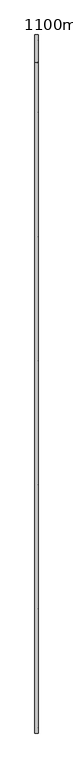
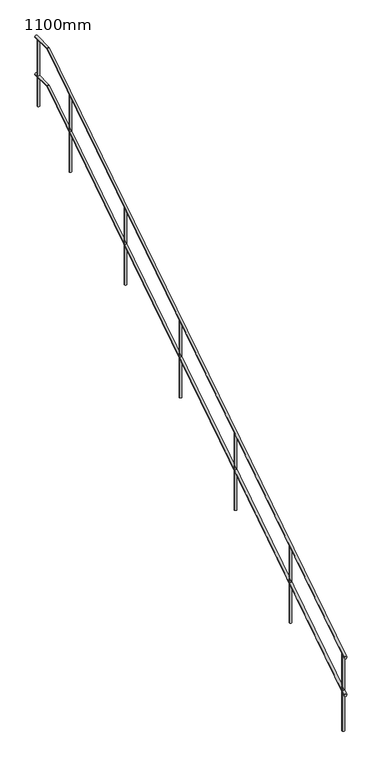
"""IFC4 building model written with IfcOpenShell, lengths in millimetres: railing geometry, 1100mm."""

import ifcopenshell
import ifcopenshell.guid

model = None  # the IFC model being written
_history = None  # IfcOwnerHistory: only IFC2X3 demands one
_inside = {}  # id of a spatial element -> (the spatial element, [elements in it])
_under = {}  # id of a project, library or spatial element -> (it, [spatial elements below it])
_declared = {}  # id of a project -> (the project, [libraries it declares])
_typed = {}  # id of a type object -> (the type object, [elements of that type])
_made_of = {}  # id of a material, layer set ... -> (it, [elements and type objects made of it])


def new_model(schema):
    """Start an empty IFC model of exactly this schema.

    Asked for "IFC4X3", IfcOpenShell would pick the latest addendum, in which some entities
    have other attributes; the version numbers below select the first issue.
    IFC2X3 requires an IfcOwnerHistory on every rooted entity: one is made here for all.
    """
    global model, _history
    if schema == "IFC4X3":
        model = ifcopenshell.file(schema_version=(4, 3, 0, 0))
    else:
        model = ifcopenshell.file(schema=schema)
    _inside.clear()
    _under.clear()
    _declared.clear()
    _typed.clear()
    _made_of.clear()
    _history = None
    if model.schema == "IFC2X3":
        org = make("IfcOrganization", Name="unknown")
        user = make(
            "IfcPersonAndOrganization",
            ThePerson=make("IfcPerson", FamilyName="unknown"),
            TheOrganization=org,
        )
        app = make(
            "IfcApplication",
            ApplicationDeveloper=org,
            Version="unknown",
            ApplicationFullName="unknown",
            ApplicationIdentifier="unknown",
        )
        _history = make(
            "IfcOwnerHistory",
            OwningUser=user,
            OwningApplication=app,
            ChangeAction="ADDED",
            CreationDate=0,
        )
    return model


def make(cls, **values):
    """One entity of the class cls with the attributes given. An attribute that is None is left unset."""
    return model.create_entity(
        cls, **{name: value for name, value in values.items() if value is not None}
    )


def rooted(cls, **values):
    """An entity with a GlobalId (a new one), such as an element, a storey or a relation."""
    return make(cls, GlobalId=ifcopenshell.guid.new(), OwnerHistory=_history, **values)


def si_unit(unit_type, name, prefix=None):
    """IfcSIUnit, for example si_unit("LENGTHUNIT", "METRE", prefix="MILLI")."""
    return make("IfcSIUnit", UnitType=unit_type, Prefix=prefix, Name=name)


def assignment(units):
    """IfcUnitAssignment: the units of a project."""
    return None if units is None else make("IfcUnitAssignment", Units=units)


def point(xyz):
    """IfcCartesianPoint."""
    return None if xyz is None else make("IfcCartesianPoint", Coordinates=xyz)


def direction(xyz):
    """IfcDirection."""
    return None if xyz is None else make("IfcDirection", DirectionRatios=xyz)


def frame(location, z_axis=None, x_axis=None):
    """IfcAxis2Placement3D, a coordinate frame: its origin and axes. An axis left out is left unset."""
    return make(
        "IfcAxis2Placement3D",
        Location=point(location),
        Axis=direction(z_axis),
        RefDirection=direction(x_axis),
    )


def frame_2d(location, x_axis=None):
    """IfcAxis2Placement2D, a coordinate frame in the plane: its origin and x axis."""
    return make(
        "IfcAxis2Placement2D", Location=point(location), RefDirection=direction(x_axis)
    )


def origin():
    """The frame at (0, 0, 0) with its axes left unset."""
    return frame((0.0, 0.0, 0.0))


def place(relative_to, where):
    """IfcLocalPlacement: puts the frame where relative to a parent placement (None: the world)."""
    return make(
        "IfcLocalPlacement", PlacementRelTo=relative_to, RelativePlacement=where
    )


def context(
    kind, dimensions, precision=None, world=None, true_north=None, identifier=None
):
    """IfcGeometricRepresentationContext, for example the 3D "Model" context."""
    return make(
        "IfcGeometricRepresentationContext",
        ContextIdentifier=identifier,
        ContextType=kind,
        CoordinateSpaceDimension=dimensions,
        Precision=precision,
        WorldCoordinateSystem=world,
        TrueNorth=true_north,
    )


def project(units=None, contexts=None):
    """IfcProject with its units and contexts."""
    return rooted(
        "IfcProject",
        Name="project",
        RepresentationContexts=contexts,
        UnitsInContext=assignment(units),
    )


def spatial(cls, under=None, at=None, **own):
    """A site, building, storey or space (cls), placed at a placement, below another one or the project."""
    s = rooted(cls, ObjectPlacement=at, **own)
    if under is not None:
        _under.setdefault(under.id(), (under, []))[1].append(s)
    return s


def circle_curve(where, radius):
    """IfcCircle in the frame where."""
    return make("IfcCircle", Position=where, Radius=radius)


def ellipse_curve(where, semi_axis1, semi_axis2):
    """IfcEllipse in the frame where."""
    return make(
        "IfcEllipse", Position=where, SemiAxis1=semi_axis1, SemiAxis2=semi_axis2
    )


def trimmed(basis, trim1, trim2, sense, master):
    """IfcTrimmedCurve: the piece of a basis curve between two trims."""
    return make(
        "IfcTrimmedCurve",
        BasisCurve=basis,
        Trim1=trim1,
        Trim2=trim2,
        SenseAgreement=sense,
        MasterRepresentation=master,
    )


def segment(curve, same_sense, transition):
    """IfcCompositeCurveSegment."""
    return make(
        "IfcCompositeCurveSegment",
        Transition=transition,
        SameSense=same_sense,
        ParentCurve=curve,
    )


def composite_curve(segments, self_intersect=None):
    """IfcCompositeCurve: segments joined end to end."""
    return make("IfcCompositeCurve", Segments=segments, SelfIntersect=self_intersect)


def outline(outer, holes=None, kind="AREA"):
    """IfcArbitraryClosedProfileDef: a profile drawn as a closed curve; with holes, ...WithVoids."""
    if holes is None:
        return make("IfcArbitraryClosedProfileDef", ProfileType=kind, OuterCurve=outer)
    return make(
        "IfcArbitraryProfileDefWithVoids",
        ProfileType=kind,
        OuterCurve=outer,
        InnerCurves=holes,
    )


def extrude(swept, where, along, depth):
    """IfcExtrudedAreaSolid: the profile swept, set in the frame where, extruded along a direction by depth."""
    return make(
        "IfcExtrudedAreaSolid",
        SweptArea=swept,
        Position=where,
        ExtrudedDirection=direction(along),
        Depth=depth,
    )


def shape(context_of_items, identifier, shape_type, items):
    """IfcShapeRepresentation: the items that make up one representation, for example the "Body"."""
    return make(
        "IfcShapeRepresentation",
        ContextOfItems=context_of_items,
        RepresentationIdentifier=identifier,
        RepresentationType=shape_type,
        Items=items,
    )


def source(mapping_origin, context_of_items, identifier, shape_type, items):
    """IfcRepresentationMap: a shape defined once, which mapped items show again and again."""
    return make(
        "IfcRepresentationMap",
        MappingOrigin=mapping_origin,
        MappedRepresentation=shape(context_of_items, identifier, shape_type, items),
    )


def transform(
    local_origin,
    x_axis=None,
    y_axis=None,
    z_axis=None,
    scale=None,
    scale2=None,
    scale3=None,
    uniform=True,
):
    """IfcCartesianTransformationOperator3D, or its non-uniform kind. x_axis, y_axis, z_axis: its Axis1, 2, 3."""
    if uniform:
        return make(
            "IfcCartesianTransformationOperator3D",
            Axis1=direction(x_axis),
            Axis2=direction(y_axis),
            LocalOrigin=point(local_origin),
            Scale=scale,
            Axis3=direction(z_axis),
        )
    return make(
        "IfcCartesianTransformationOperator3DnonUniform",
        Axis1=direction(x_axis),
        Axis2=direction(y_axis),
        LocalOrigin=point(local_origin),
        Scale=scale,
        Axis3=direction(z_axis),
        Scale2=scale2,
        Scale3=scale3,
    )


def mapped(mapping_source, mapping_target):
    """IfcMappedItem: shows the shape of a source again, moved by a transform."""
    return make(
        "IfcMappedItem", MappingSource=mapping_source, MappingTarget=mapping_target
    )


def made_of(thing, what):
    """Note that an element or type object is made of a material, layer set ...; save() writes the relation."""
    if what is not None:
        _made_of.setdefault(what.id(), (what, []))[1].append(thing)
    return thing


def element(
    cls,
    number,
    at=None,
    inside=None,
    cuts=None,
    type_object=None,
    material=None,
    context=None,
    identifier="Body",
    shape_type=None,
    held_by="IfcProductDefinitionShape",
    body=None,
    shapes=None,
    **own,
):
    """One element of the class cls, such as IfcWall. Its Tag is "e" and its number.

    at: its placement. inside: the storey or other place that contains it. cuts: it is an
    opening in that element (IfcRelVoidsElement). A single representation is given by context,
    identifier, shape_type and body (its items); several are given by shapes. held_by: the class
    of the entity that holds the representations. save() writes the other relations.
    """
    e = rooted(cls, Tag="e%d" % number, ObjectPlacement=at, **own)
    if body is not None:
        shapes = [shape(context, identifier, shape_type, body)]
    if shapes is not None:
        e.Representation = make(held_by, Representations=shapes)
    if inside is not None:
        _inside.setdefault(inside.id(), (inside, []))[1].append(e)
    if cuts is not None:
        rooted(
            "IfcRelVoidsElement", RelatingBuildingElement=cuts, RelatedOpeningElement=e
        )
    if type_object is not None:
        _typed.setdefault(type_object.id(), (type_object, []))[1].append(e)
    return made_of(e, material)


def aggregate(whole, parts):
    """IfcRelAggregates: a whole, such as a stair, and the parts it consists of."""
    return rooted("IfcRelAggregates", RelatingObject=whole, RelatedObjects=parts)


def save(model, path):
    """Write the relations noted so far, then the file.

    IfcRelAggregates (storeys below a building ...), IfcRelContainedInSpatialStructure (elements
    in a storey), IfcRelDefinesByType, IfcRelAssociatesMaterial and IfcRelDeclares: one each for
    every whole, place, type object, material and project.
    """
    for whole, parts in _under.values():
        aggregate(whole, parts)
    for where, things in _inside.values():
        rooted(
            "IfcRelContainedInSpatialStructure",
            RelatedElements=things,
            RelatingStructure=where,
        )
    for kind, things in _typed.values():
        rooted("IfcRelDefinesByType", RelatedObjects=things, RelatingType=kind)
    for what, things in _made_of.values():
        rooted("IfcRelAssociatesMaterial", RelatedObjects=things, RelatingMaterial=what)
    for by, libraries in _declared.values():
        rooted("IfcRelDeclares", RelatingContext=by, RelatedDefinitions=libraries)
    model.write(path)


def plane_surface(at):
    """IfcPlane: the flat surface through the origin of the frame at, square to its z axis."""
    return make("IfcPlane", Position=at)


def cylinder_surface(at, radius):
    """IfcCylindricalSurface: all points at the distance radius from the z axis of the frame at."""
    return make("IfcCylindricalSurface", Position=at, Radius=radius)


def advanced_brep(points, edges, surfaces, faces):
    """IfcAdvancedBrep: a solid bounded by faces that lie on surfaces and meet in shared edges.

    An edge is (start, end): straight between two places in points (the first is 0);
    or (start, end, curve); or (start, end, curve, False) where it runs against its curve.
    A face is (place in surfaces, loops), or (place, loops, False) where it looks against
    its surface's normal. A loop lists edges by number (the first is 1), with a minus sign
    where the edge is run from its end to its start. The first loop is the outer one.
    """
    corners = [point(p) for p in points]
    vertices = [make("IfcVertexPoint", VertexGeometry=c) for c in corners]
    made = []
    for start, end, *more in edges:
        made.append(
            make(
                "IfcEdgeCurve",
                EdgeStart=vertices[start],
                EdgeEnd=vertices[end],
                EdgeGeometry=more[0] if more else make("IfcPolyline", Points=[corners[start], corners[end]]),
                SameSense=more[1] if len(more) > 1 else True,
            )
        )
    hull = []
    for where, loops, *sense in faces:
        bounds = []
        for j, loop in enumerate(loops):
            ring = [make("IfcOrientedEdge", EdgeElement=made[abs(k) - 1], Orientation=k > 0) for k in loop]
            bounds.append(
                make(
                    "IfcFaceOuterBound" if j == 0 else "IfcFaceBound",
                    Bound=make("IfcEdgeLoop", EdgeList=ring),
                    Orientation=True,
                )
            )
        hull.append(make("IfcAdvancedFace", Bounds=bounds, FaceSurface=surfaces[where], SameSense=sense[0] if sense else True))
    return make("IfcAdvancedBrep", Outer=make("IfcClosedShell", CfsFaces=hull))


def railing_1100mm_756f1f54(model_context):
    return source(origin(), model_context, "Body", "SolidModel", [
        advanced_brep(
        [(17846.6097182, 11187.7630152, 456.1549882), (17816.6097182, 11187.7630152, 456.1549882), (17846.6097182, 17937.7630152, 4635.0), (17816.6097182, 17937.7630152, 4635.0), (17846.6097182, 17672.1776886, 4635.0), (17816.6097182, 17672.1776886, 4635.0)],
        [
            (0, 1, ellipse_curve(frame((17831.6097182, 11187.7630152, 456.1549882), z_axis=(0.0, -1.0, 0.0), x_axis=(0.0, 0.0, -1.0)), 17.8450118, 15.0)),
            (1, 0, ellipse_curve(frame((17831.6097182, 11187.7630152, 456.1549882), z_axis=(0.0, -1.0, 0.0), x_axis=(0.0, 0.0, -1.0)), 17.8450118, 15.0)),
            (2, 3, circle_curve(frame((17831.6097182, 17937.7630152, 4635.0), z_axis=(0.0, 1.0, 0.0), x_axis=(-1.0, 0.0, 0.0)), 15.0)),
            (3, 2, circle_curve(frame((17831.6097182, 17937.7630152, 4635.0), z_axis=(0.0, 1.0, 0.0), x_axis=(-1.0, 0.0, 0.0)), 15.0)),
            (0, 4),
            (4, 5, ellipse_curve(frame((17831.6097182, 17672.1776886, 4635.0), z_axis=(0.0, -0.9593151294266218, -0.28233753284532276), x_axis=(0.0, 0.282337532845322, -0.9593151294266221)), 15.6361549, 15.0)),
            (5, 1),
            (5, 4, ellipse_curve(frame((17831.6097182, 17672.1776886, 4635.0), z_axis=(0.0, -0.9593151294266218, -0.28233753284532276), x_axis=(0.0, 0.282337532845322, -0.9593151294266221)), 15.6361549, 15.0)),
            (4, 2),
            (3, 5),
        ],
        [
            plane_surface(frame((17831.6097182, 11187.7630152, 474.0), z_axis=(0.0, -1.0, 0.0), x_axis=(0.0, 0.0, 1.0))),
            plane_surface(frame((17831.6097182, 17937.7630152, 4650.0), z_axis=(0.0, 1.0, 0.0), x_axis=(0.0, 0.0, 1.0))),
            cylinder_surface(frame((17831.6097182, 11195.8885352, 461.3914345), z_axis=(0.0, -0.8405710350936326, -0.5417013337270078), x_axis=(-1.0, 0.0, 0.0)), 15.0),
            cylinder_surface(frame((17831.6097182, 17667.7630152, 4635.0), z_axis=(0.0, -1.0, 0.0), x_axis=(-1.0, 0.0, 0.0)), 15.0),
        ],
        [
            (0, [[1, 2]]),
            (1, [[3, 4]]),
            (2, [[-1, 5, 6, 7]]),
            (2, [[-2, -7, 8, -5]]),
            (3, [[-6, 9, -4, 10]]),
            (3, [[-8, -10, -3, -9]]),
        ],
    ),
        advanced_brep(
        [(17846.6097182, 11187.7630152, 956.1549882), (17816.6097182, 11187.7630152, 956.1549882), (17846.6097182, 17672.1776886, 5135.0), (17816.6097182, 17672.1776886, 5135.0), (17846.6097182, 17937.7630152, 5135.0), (17816.6097182, 17937.7630152, 5135.0)],
        [
            (0, 1, ellipse_curve(frame((17831.6097182, 11187.7630152, 956.1549882), z_axis=(0.0, -1.0, 0.0), x_axis=(0.0, 0.0, -1.0)), 17.8450118, 15.0)),
            (1, 0, ellipse_curve(frame((17831.6097182, 11187.7630152, 956.1549882), z_axis=(0.0, -1.0, 0.0), x_axis=(0.0, 0.0, -1.0)), 17.8450118, 15.0)),
            (0, 2),
            (2, 3, ellipse_curve(frame((17831.6097182, 17672.1776886, 5135.0), z_axis=(0.0, -0.9593151294266218, -0.28233753284532276), x_axis=(0.0, 0.282337532845322, -0.9593151294266221)), 15.6361549, 15.0)),
            (3, 1),
            (3, 2, ellipse_curve(frame((17831.6097182, 17672.1776886, 5135.0), z_axis=(0.0, -0.9593151294266218, -0.28233753284532276), x_axis=(0.0, 0.282337532845322, -0.9593151294266221)), 15.6361549, 15.0)),
            (4, 5, circle_curve(frame((17831.6097182, 17937.7630152, 5135.0), z_axis=(0.0, 1.0, 0.0), x_axis=(-1.0, 0.0, 0.0)), 15.0)),
            (5, 4, circle_curve(frame((17831.6097182, 17937.7630152, 5135.0), z_axis=(0.0, 1.0, 0.0), x_axis=(-1.0, 0.0, 0.0)), 15.0)),
            (2, 4),
            (5, 3),
        ],
        [
            plane_surface(frame((17831.6097182, 11187.7630152, 974.0), z_axis=(0.0, -1.0, 0.0), x_axis=(0.0, 0.0, 1.0))),
            cylinder_surface(frame((17831.6097182, 11195.8885352, 961.3914345), z_axis=(0.0, -0.8405710350936326, -0.5417013337270078), x_axis=(-1.0, 0.0, 0.0)), 15.0),
            plane_surface(frame((17831.6097182, 17937.7630152, 5150.0), z_axis=(0.0, 1.0, 0.0), x_axis=(0.0, 0.0, 1.0))),
            cylinder_surface(frame((17831.6097182, 17667.7630152, 5135.0), z_axis=(0.0, -1.0, 0.0), x_axis=(-1.0, 0.0, 0.0)), 15.0),
        ],
        [
            (0, [[1, 2]]),
            (1, [[-1, 3, 4, 5]]),
            (1, [[-2, -5, 6, -3]]),
            (2, [[7, 8]]),
            (3, [[-4, 9, -8, 10]]),
            (3, [[-6, -10, -7, -9]]),
        ],
    ),
        extrude(outline(composite_curve([segment(trimmed(circle_curve(frame_2d((17831.6097182, 17187.7630152)), 15.0), [point((17816.6097182, 17187.7630152))], [point((17846.6097182, 17187.7630152))], False, "CARTESIAN"), True, "CONTINUOUS"), segment(trimmed(circle_curve(frame_2d((17831.6097182, 17187.7630152)), 15.0), [point((17846.6097182, 17187.7630152))], [point((17816.6097182, 17187.7630152))], False, "CARTESIAN"), True, "CONTINUOUS")], self_intersect=False)), frame((0.0, 0.0, 3790.4451685), z_axis=(0.0, 0.0, 1.0), x_axis=(1.0, 0.0, 0.0)), (0.0, 0.0, 1.0), 1020.2214982),
        extrude(outline(composite_curve([segment(trimmed(circle_curve(frame_2d((17831.6097182, 15987.7630152)), 15.0), [point((17816.6097182, 15987.7630152))], [point((17846.6097182, 15987.7630152))], False, "CARTESIAN"), True, "CONTINUOUS"), segment(trimmed(circle_curve(frame_2d((17831.6097182, 15987.7630152)), 15.0), [point((17846.6097182, 15987.7630152))], [point((17816.6097182, 15987.7630152))], False, "CARTESIAN"), True, "CONTINUOUS")], self_intersect=False)), frame((0.0, 0.0, 3017.1118351), z_axis=(0.0, 0.0, 1.0), x_axis=(1.0, 0.0, 0.0)), (0.0, 0.0, 1.0), 1020.2214982),
        extrude(outline(composite_curve([segment(trimmed(circle_curve(frame_2d((17831.6097182, 14787.7630152)), 15.0), [point((17816.6097182, 14787.7630152))], [point((17846.6097182, 14787.7630152))], False, "CARTESIAN"), True, "CONTINUOUS"), segment(trimmed(circle_curve(frame_2d((17831.6097182, 14787.7630152)), 15.0), [point((17846.6097182, 14787.7630152))], [point((17816.6097182, 14787.7630152))], False, "CARTESIAN"), True, "CONTINUOUS")], self_intersect=False)), frame((0.0, 0.0, 2243.7785018), z_axis=(0.0, 0.0, 1.0), x_axis=(1.0, 0.0, 0.0)), (0.0, 0.0, 1.0), 1020.2214982),
        extrude(outline(composite_curve([segment(trimmed(circle_curve(frame_2d((17831.6097182, 13587.7630152)), 15.0), [point((17816.6097182, 13587.7630152))], [point((17846.6097182, 13587.7630152))], False, "CARTESIAN"), True, "CONTINUOUS"), segment(trimmed(circle_curve(frame_2d((17831.6097182, 13587.7630152)), 15.0), [point((17846.6097182, 13587.7630152))], [point((17816.6097182, 13587.7630152))], False, "CARTESIAN"), True, "CONTINUOUS")], self_intersect=False)), frame((0.0, 0.0, 1470.4451685), z_axis=(0.0, 0.0, 1.0), x_axis=(1.0, 0.0, 0.0)), (0.0, 0.0, 1.0), 1020.2214982),
        extrude(outline(composite_curve([segment(trimmed(circle_curve(frame_2d((17831.6097182, 12387.7630152)), 15.0), [point((17816.6097182, 12387.7630152))], [point((17846.6097182, 12387.7630152))], False, "CARTESIAN"), True, "CONTINUOUS"), segment(trimmed(circle_curve(frame_2d((17831.6097182, 12387.7630152)), 15.0), [point((17846.6097182, 12387.7630152))], [point((17816.6097182, 12387.7630152))], False, "CARTESIAN"), True, "CONTINUOUS")], self_intersect=False)), frame((0.0, 0.0, 697.1118351), z_axis=(0.0, 0.0, 1.0), x_axis=(1.0, 0.0, 0.0)), (0.0, 0.0, 1.0), 1020.2214982),
        extrude(outline(composite_curve([segment(trimmed(circle_curve(frame_2d((17831.6097182, 17887.7630152)), 15.0), [point((17816.6097182, 17887.7630152))], [point((17846.6097182, 17887.7630152))], False, "CARTESIAN"), True, "CONTINUOUS"), segment(trimmed(circle_curve(frame_2d((17831.6097182, 17887.7630152)), 15.0), [point((17846.6097182, 17887.7630152))], [point((17816.6097182, 17887.7630152))], False, "CARTESIAN"), True, "CONTINUOUS")], self_intersect=False)), frame((0.0, 0.0, 4241.5562796), z_axis=(0.0, 0.0, 1.0), x_axis=(1.0, 0.0, 0.0)), (0.0, 0.0, 1.0), 878.4437204),
        extrude(outline(composite_curve([segment(trimmed(circle_curve(frame_2d((17831.6097182, 11237.7630152)), 15.0), [point((17816.6097182, 11237.7630152))], [point((17846.6097182, 11237.7630152))], False, "CARTESIAN"), True, "CONTINUOUS"), segment(trimmed(circle_curve(frame_2d((17831.6097182, 11237.7630152)), 15.0), [point((17846.6097182, 11237.7630152))], [point((17816.6097182, 11237.7630152))], False, "CARTESIAN"), True, "CONTINUOUS")], self_intersect=False)), frame((0.0, 0.0, -43.999276), z_axis=(0.0, 0.0, 1.0), x_axis=(1.0, 0.0, 0.0)), (0.0, 0.0, 1.0), 1020.2214982),
    ])


if __name__ == "__main__":
    model = new_model("IFC4")
    model_context = context("Model", 3, world=origin())
    ifc_project = project(units=[si_unit("LENGTHUNIT", "METRE", prefix="MILLI")], contexts=[model_context])
    site = spatial("IfcSite", under=ifc_project)
    building = spatial("IfcBuilding", under=site)
    placement = place(None, origin())
    railing_1100mm_shape = railing_1100mm_756f1f54(model_context)
    element("IfcRailing", 1, ObjectType="1100mm", at=placement, inside=building, context=model_context, shape_type="MappedRepresentation", body=[
        mapped(railing_1100mm_shape, transform((0.0, 0.0, 0.0), x_axis=(1.0, 0.0, 0.0), y_axis=(0.0, 1.0, 0.0), z_axis=(0.0, 0.0, 1.0))),
    ])
    save(model, "model.ifc")
